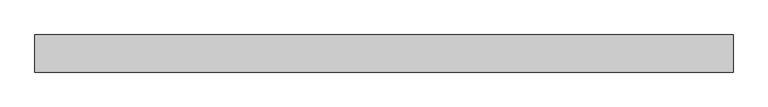
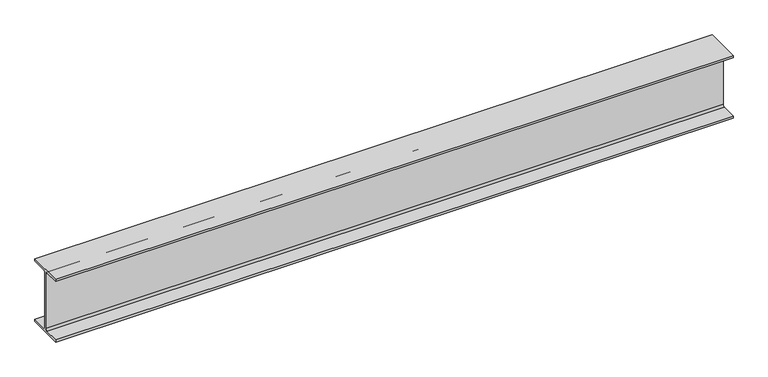
"""IFC4 building model written with IfcOpenShell, lengths in millimetres: beam geometry, Old_Steel Beam_H-KSD3502 : H_SB_ASB_H-200×200x8x12."""

from ifc_helpers import new_model, si_unit, point, frame, frame_2d, origin, place, context, project, spatial, polyline, circle_curve, trimmed, segment, composite_curve, outline, extrude, source, transform, mapped, element, save


def beam_c9ddaae5(model_context):
    return source(origin(), model_context, "Body", "SweptSolid", [
        extrude(outline(composite_curve([segment(polyline([(82.5, -141.5), (82.5, -151.7), (-82.5, -151.7), (-82.5, -141.5), (-11.9, -141.5)]), True, "CONTINUOUS"), segment(trimmed(circle_curve(frame_2d((-11.9, -132.6)), 8.9), [point((-11.9, -141.5))], [point((-3.0, -132.6))], True, "CARTESIAN"), True, "CONTINUOUS"), segment(polyline([(-3.0, -132.6), (-3.0, 132.6)]), True, "CONTINUOUS"), segment(trimmed(circle_curve(frame_2d((-11.9, 132.6)), 8.9), [point((-3.0, 132.6))], [point((-11.9, 141.5))], True, "CARTESIAN"), True, "CONTINUOUS"), segment(polyline([(-11.9, 141.5), (-82.5, 141.5), (-82.5, 151.7), (82.5, 151.7), (82.5, 141.5), (11.9, 141.5)]), True, "CONTINUOUS"), segment(trimmed(circle_curve(frame_2d((11.9, 132.6)), 8.9), [point((11.9, 141.5))], [point((3.0, 132.6))], True, "CARTESIAN"), True, "CONTINUOUS"), segment(polyline([(3.0, 132.6), (3.0, -132.6)]), True, "CONTINUOUS"), segment(trimmed(circle_curve(frame_2d((11.9, -132.6)), 8.9), [point((3.0, -132.6))], [point((11.9, -141.5))], True, "CARTESIAN"), True, "CONTINUOUS"), segment(polyline([(11.9, -141.5), (82.5, -141.5)]), True, "CONTINUOUS")], self_intersect=False)), frame((-1380.4746851, 0.0, 0.0), z_axis=(1.0, 0.0, 0.0), x_axis=(0.0, 1.0, 0.0)), (0.0, 0.0, 1.0), 3103.2859215),
    ])


if __name__ == "__main__":
    model = new_model("IFC4")
    model_context = context("Model", 3, world=origin())
    ifc_project = project(units=[si_unit("LENGTHUNIT", "METRE", prefix="MILLI")], contexts=[model_context])
    site = spatial("IfcSite", under=ifc_project)
    building = spatial("IfcBuilding", under=site)
    placement = place(None, origin())
    beam_shape = beam_c9ddaae5(model_context)
    element("IfcBeam", 1, ObjectType="Old_Steel Beam_H-KSD3502 : H_SB_ASB_H-200×200x8x12", at=placement, inside=building, context=model_context, shape_type="MappedRepresentation", body=[
        mapped(beam_shape, transform((0.0, 0.0, 0.0), x_axis=(1.0, 0.0, 0.0), y_axis=(0.0, 1.0, 0.0), z_axis=(0.0, 0.0, 1.0))),
    ])
    save(model, "model.ifc")

# Revit data of these elements
# Type "Old_Steel Beam_H-KSD3502 : H_SB_ASB_H-200×200x8x12"
#   Width = 20.0 cm
#   Web Thickness = 0.8 cm
#   Web Fillet = 1.3 cm
#   Warping Constant = 141376.0 cm⁶
#   Torsional Moment of Inertia = 26.2485 cm⁴
#   Torsional Modulus = 1.0 cm³
#   Section Area = 63.53 cm²
#   Plastic Modulus weak axis = 244.0 cm³
#   Plastic Modulus strong axis = 525.0 cm³
#   Perimeter = 1.16 m²/m
#   Nominal Weight = 49.90 kgf/m
#   Moment of Inertia weak axis = 1600.00 cm⁴
#   Moment of Inertia strong axis = 4720.00 cm⁴
#   Height = 20.0 cm
#   Flange Thickness = 1.2 cm
#   Elastic Modulus weak axis = 160.0 cm³
#   Elastic Modulus strong axis = 472.0 cm³
#   Centroid Vertical = 10.0 cm
#   Centroid Horizontal = 10.0 cm
#   Length [instance default] = 1.5240 m
#   Structural Material [instance default] = Steel, 45-345
#   Assembly Code = ""
# Element 1 (IfcBeam, "Old_Steel Beam_H-KSD3502 : H_SB_ASB_H-200×200x8x12")
#   Structural Material = none
# Materials
#   "Steel, 45-345": class "Metal", colour RGB 189 187 185, transparency 0, Description = "Steel 345 MPa", Cost = 0
